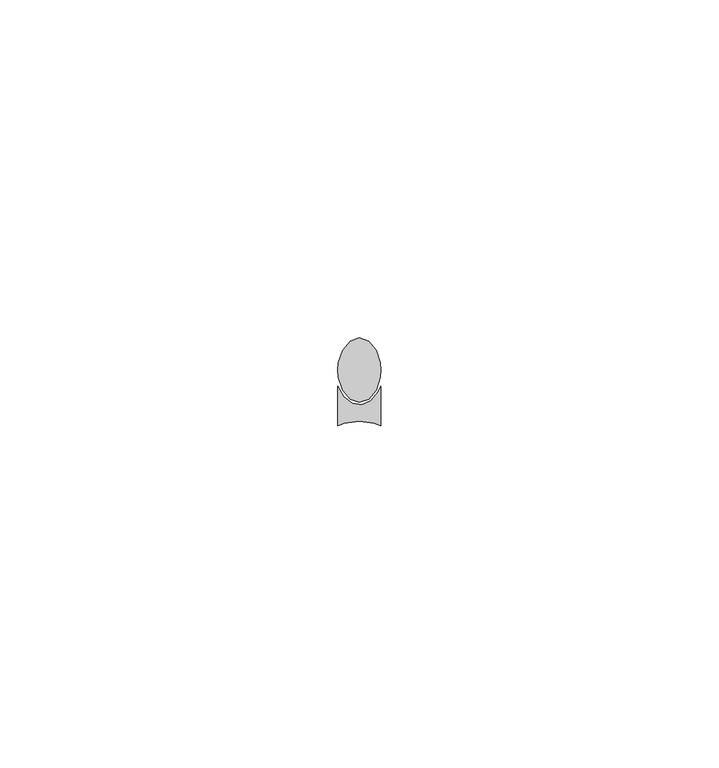
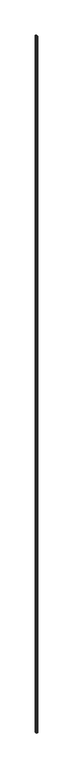
"""IFC4 building model written with IfcOpenShell, lengths in millimetres: proxy geometry, Generic Models 11:Generic Models 1:306267:Generic Models 1:306267 : Generic Models 11:Generic Models 1:306267:300405:Generic Models 1:306267:Generic Models 1:306267 : Generic Models 11:Generic Models 1:306267:300405 : Generic Models 11:Generic Models 1:306267:Generic Models 1:306267 : Generic Models 11:Generic Models 1:306267:300405:15 : Generic Models 11:Generic Models 1:306267:Generic Models 1:306267 : Generic Models 11:Generic Models 1:306267:300405:Generic Models 1:306267:Generic Models 1:306267 : Generic Models 11:Generic Models 1:306267:300405 : Generic Models 11:Generic Models 1:306267:Generic Models 1:306267 : Generic Models 11:Generic Models 1:306267:300405:300182."""

from ifc_helpers import new_model, si_unit, origin, origin_with_axes, place, context, project, spatial, polyline, outline, extrude, source, transform, mapped, element, save


def generic_models_3c596d45(model_context):
    return source(origin(), model_context, "Body", "SweptSolid", [
        extrude(outline(polyline([(582706.3393048, -579082.4586403), (582704.9617239, -579082.9302761), (582703.5841431, -579082.4586403), (582702.479409, -579081.1371463), (582701.8663278, -579079.2275321), (582701.7867239, -579078.1677761), (582701.8663278, -579077.1080202), (582702.479409, -579075.1984059), (582703.5841431, -579073.8769119), (582704.9617239, -579073.4052761), (582706.3393048, -579073.8769119), (582707.4440389, -579075.1984059), (582708.0571201, -579077.1080202), (582708.1367239, -579078.1677761), (582708.0571201, -579079.2275321), (582707.4440389, -579081.1371463), (582706.3393048, -579082.4586403)])), origin_with_axes(), (0.0, 0.0, 1.0), 3695.7),
        extrude(outline(polyline([(582702.7524872, -579086.0220872), (582701.7867239, -579086.3994958), (582701.7867239, -579080.5314037), (582702.6695128, -579082.1246204), (582703.9108969, -579083.0988254), (582705.3166731, -579083.3016133), (582706.6669209, -579082.7012598), (582707.7504064, -579081.3916847), (582708.1367239, -579080.5314037), (582708.1367239, -579086.3994958), (582707.1709607, -579086.0220872), (582704.9617239, -579085.7084011), (582702.7524872, -579086.0220872)])), origin_with_axes(), (0.0, 0.0, 1.0), 3695.7),
    ])


if __name__ == "__main__":
    model = new_model("IFC4")
    model_context = context("Model", 3, world=origin())
    ifc_project = project(units=[si_unit("LENGTHUNIT", "METRE", prefix="MILLI")], contexts=[model_context])
    site = spatial("IfcSite", under=ifc_project)
    building = spatial("IfcBuilding", under=site)
    placement = place(None, origin())
    generic_models_shape = generic_models_3c596d45(model_context)
    element("IfcBuildingElementProxy", 1, Name="Generic Models 11:Generic Models 1:306267:Generic Models 1:306267 : Generic Models 11:Generic Models 1:306267:300405:Generic Models 1:306267:Generic Models 1:306267 : Generic Models 11:Generic Models 1:306267:300405 : Generic Models 11:Generic Models 1:306267:Generic Models 1:306267 : Generic Models 11:Generic Models 1:306267:300405:15 : Generic Models 11:Generic Models 1:306267:Generic Models 1:306267 : Generic Models 11:Generic Models 1:306267:300405:Generic Models 1:306267:Generic Models 1:306267 : Generic Models 11:Generic Models 1:306267:300405 : Generic Models 11:Generic Models 1:306267:Generic Models 1:306267 : Generic Models 11:Generic Models 1:306267:300405:300182", ObjectType="Generic Models 11:Generic Models 1:306267:Generic Models 1:306267 : Generic Models 11:Generic Models 1:306267:300405:Generic Models 1:306267:Generic Models 1:306267 : Generic Models 11:Generic Models 1:306267:300405 : Generic Models 11:Generic Models 1:306267:Generic Models 1:306267 : Generic Models 11:Generic Models 1:306267:300405:15 : Generic Models 11:Generic Models 1:306267:Generic Models 1:306267 : Generic Models 11:Generic Models 1:306267:300405:Generic Models 1:306267:Generic Models 1:306267 : Generic Models 11:Generic Models 1:306267:300405 : Generic Models 11:Generic Models 1:306267:Generic Models 1:306267 : Generic Models 11:Generic Models 1:306267:300405:300182", at=placement, inside=building, context=model_context, shape_type="MappedRepresentation", body=[
        mapped(generic_models_shape, transform((0.0, 0.0, 0.0), x_axis=(1.0, 0.0, 0.0), y_axis=(0.0, 1.0, 0.0), z_axis=(0.0, 0.0, 1.0))),
    ])
    save(model, "model.ifc")

# Revit data of these elements
# Type "Generic Models 11:Generic Models 1:306267:Generic Models 1:306267 : Generic Models 11:Generic Models 1:306267:300405:Generic Models 1:306267:Generic Models 1:306267 : Generic Models 11:Generic Models 1:306267:300405 : Generic Models 11:Generic Models 1:306267:Generic Models 1:306267 : Generic Models 11:Generic Models 1:306267:300405:15 : Generic Models 11:Generic Models 1:306267:Generic Models 1:306267 : Generic Models 11:Generic Models 1:306267:300405:Generic Models 1:306267:Generic Models 1:306267 : Generic Models 11:Generic Models 1:306267:300405 : Generic Models 11:Generic Models 1:306267:Generic Models 1:306267 : Generic Models 11:Generic Models 1:306267:300405:300182"
#   NameOverride = "Generic Models 11:Generic Models 1:306267:Generic Models 1:306267 : Generic Models 11:Generic Models 1:306267:300405:Generic Models 1:306267:Generic Models 1:306267 : Generic Models 11:Generic Models 1:306267:300405 : Generic Models 11:Generic Models 1:306267:Generic Models 1:306267 : Generic Models 11:Generic Models 1:306267:300405:300182"
#   ObjectTypeOverride = "Generic Models 1:306267:Generic Models 1:306267 : Generic Models 11:Generic Models 1:306267:300405 : Generic Models 11:Generic Models 1:306267:Generic Models 1:306267 : Generic Models 11:Generic Models 1:306267:300405"
#   Reference = "Generic Models 1"
#   Tag = "300182"
# Element 1 (IfcBuildingElementProxy, "Generic Models 11:Generic Models 1:306267:Generic Models 1:306267 : Generic Models 11:Generic Models 1:306267:300405:Generic Models 1:306267:Generic Models 1:306267 : Generic Models 11:Generic Models 1:306267:300405 : Generic Models 11:Generic Models 1:306267:Generic Models 1:306267 : Generic Models 11:Generic Models 1:306267:300405:15 : Generic Models 11:Generic Models 1:306267:Generic Models 1:306267 : Generic Models 11:Generic Models 1:306267:300405:Generic Models 1:306267:Generic Models 1:306267 : Generic Models 11:Generic Models 1:306267:300405 : Generic Models 11:Generic Models 1:306267:Generic Models 1:306267 : Generic Models 11:Generic Models 1:306267:300405:300182")
#   Materials on its faces: "SEALANT & BACKER ROD"
# Materials
#   "SEALANT & BACKER ROD": class "Unassigned", colour RGB 120 120 120, transparency 0, Cost = 0
